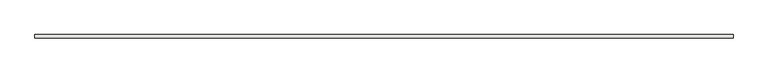
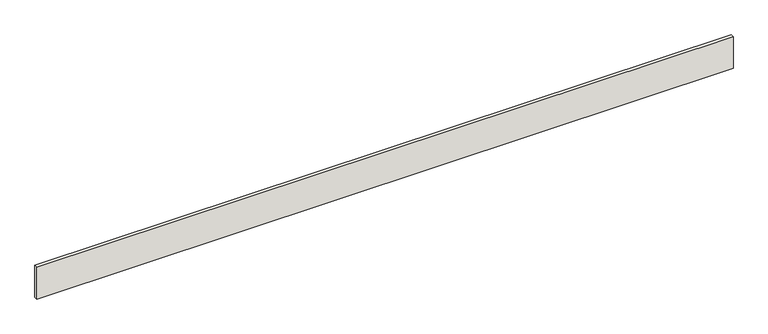
"""IFC4 building model written with IfcOpenShell, lengths in millimetres: wall geometry, Holzwand."""

from ifc_helpers import new_model, si_unit, origin, origin_with_axes, place, context, project, spatial, polyline, outline, extrude, source, transform, mapped, element, save


def wall_7fe27200(model_context):
    return source(origin(), model_context, "Body", "SweptSolid", [
        extrude(outline(polyline([(0.0, 100.0), (20802.8619019, 100.0), (20802.8619019, 0.0), (0.0, 0.0), (0.0, 100.0)])), origin_with_axes(), (0.0, 0.0, 1.0), 1000.0),
    ])


if __name__ == "__main__":
    model = new_model("IFC4")
    model_context = context("Model", 3, world=origin())
    ifc_project = project(units=[si_unit("LENGTHUNIT", "METRE", prefix="MILLI")], contexts=[model_context])
    site = spatial("IfcSite", under=ifc_project)
    building = spatial("IfcBuilding", under=site)
    placement = place(None, origin())
    wall_shape = wall_7fe27200(model_context)
    element("IfcWall", 1, ObjectType="Holzwand", at=placement, inside=building, context=model_context, shape_type="MappedRepresentation", body=[
        mapped(wall_shape, transform((0.0, 0.0, 0.0), x_axis=(1.0, 0.0, 0.0), y_axis=(0.0, 1.0, 0.0), z_axis=(0.0, 0.0, 1.0))),
    ])
    save(model, "model.ifc")

# Revit data of these elements
# Element 1 (IfcWall, "Holzwand")
#   Materials on its faces: "pv - panel anthrazit"
# Materials
#   "pv - panel anthrazit": class "Unassigned", colour RGB 128 128 128, transparency 0
